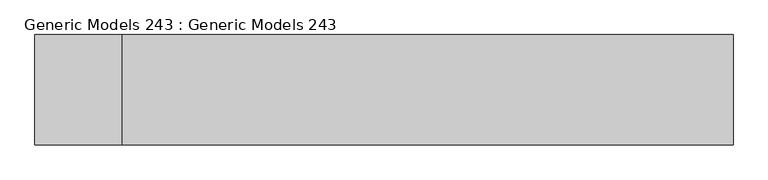
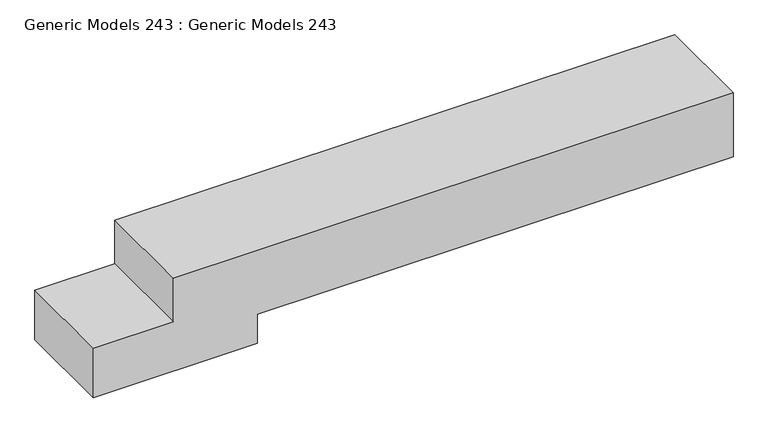
"""IFC4 building model written with IfcOpenShell, lengths in millimetres: proxy geometry, Generic Models 243 : Generic Models 243."""

from ifc_helpers import new_model, si_unit, frame, origin, place, context, project, spatial, polyline, outline, extrude, source, transform, mapped, element, save


def generic_models_243_generic_models_243_7b48a9a8(model_context):
    return source(origin(), model_context, "Body", "SweptSolid", [
        extrude(outline(polyline([(123435.8085, -63.6736296), (123297.696, -63.6736296), (123297.696, -304.9736296), (123138.946, -304.9736296), (123138.946, 190.3263704), (123232.6085, 190.3263704), (123232.6085, 1625.4263704), (123435.8085, 1625.4263704), (123435.8085, -63.6736296)])), frame((0.0, 4260.0872686, 0.0), z_axis=(0.0, 1.0, 0.0), x_axis=(0.0, 0.0, 1.0)), (0.0, 0.0, 1.0), 304.8),
    ])


if __name__ == "__main__":
    model = new_model("IFC4")
    model_context = context("Model", 3, world=origin())
    ifc_project = project(units=[si_unit("LENGTHUNIT", "METRE", prefix="MILLI")], contexts=[model_context])
    site = spatial("IfcSite", under=ifc_project)
    building = spatial("IfcBuilding", under=site)
    placement = place(None, origin())
    generic_models_243_generic_models_243_shape = generic_models_243_generic_models_243_7b48a9a8(model_context)
    element("IfcBuildingElementProxy", 1, Name="Generic Models 243 : Generic Models 243", ObjectType="Generic Models 243 : Generic Models 243", at=placement, inside=building, context=model_context, shape_type="MappedRepresentation", body=[
        mapped(generic_models_243_generic_models_243_shape, transform((0.0, 0.0, 0.0), x_axis=(1.0, 0.0, 0.0), y_axis=(0.0, 1.0, 0.0), z_axis=(0.0, 0.0, 1.0))),
    ])
    save(model, "model.ifc")

# Revit data of these elements
# Element 1 (IfcBuildingElementProxy, "Generic Models 243 : Generic Models 243")
#   Materials on its faces: "_ 8\" CONCRETE SLAB W/ GRADE BEAM (SEE STRUCT. DWGS)"
# Materials
#   "_ 8\" CONCRETE SLAB W/ GRADE BEAM (SEE STRUCT. DWGS)": class "Generic", colour RGB 191 191 191, transparency 0, Cost = 0
